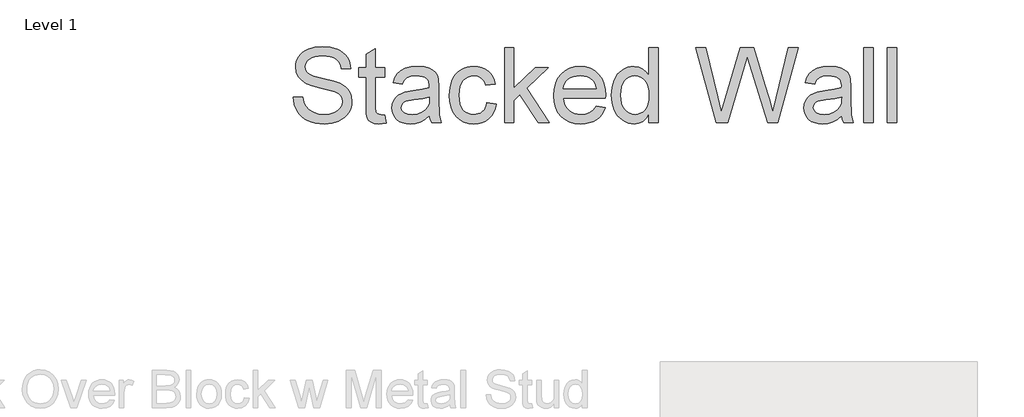
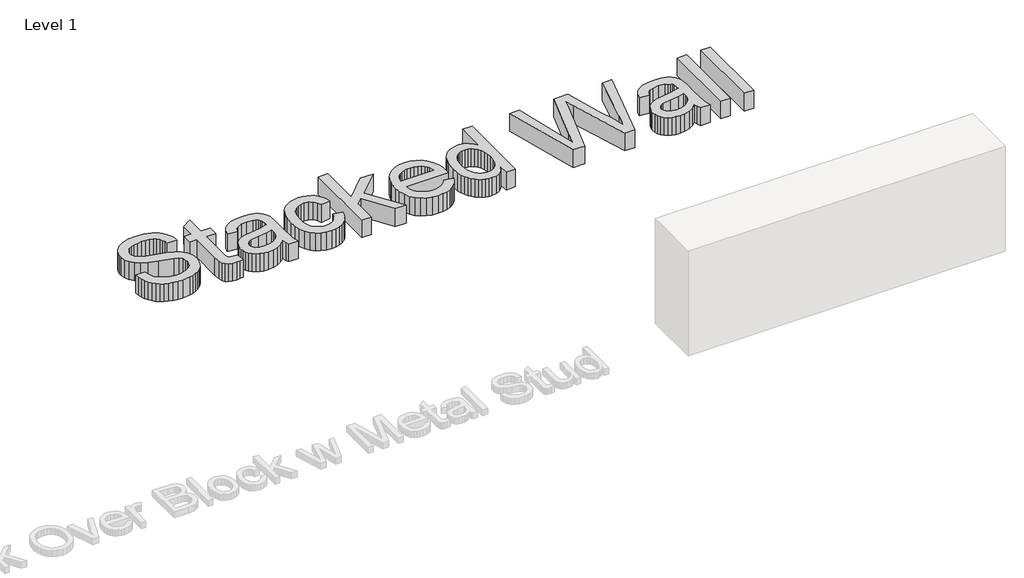
# One storey, part 42 of 42: 1 proxy.
"""IFC4 building model written with IfcOpenShell, lengths in millimetres."""

from ifc_helpers import new_model, si_unit, origin, origin_with_axes, place, context, project, spatial, polyline, outline, extrude, element, save

model = new_model("IFC4")

# Units and contexts
model_context = context("Model", 3, world=origin())
ifc_project = project(units=[si_unit("LENGTHUNIT", "METRE", prefix="MILLI")], contexts=[model_context])

# Site, building, storey
site = spatial("IfcSite", under=ifc_project)
building = spatial("IfcBuilding", under=site)
storey = spatial("IfcBuildingStorey", under=building, Name="Level 1", Elevation=0.0)

# Proxy
placement = place(None, origin())
element("IfcBuildingElementProxy", 1, Name="24\" Arial", ObjectType="24\" Arial", at=placement, inside=storey, context=model_context, shape_type="SweptSolid", body=[
    extrude(outline(polyline([(32520.8544204, 19214.0234856), (32596.9961939, 19214.0234856), (32605.733165, 19171.7700063), (32621.5340701, 19137.8073549), (32646.1834821, 19110.8528696), (32681.4659739, 19089.6238888), (32724.5931503, 19075.8492174), (32772.7766163, 19071.2576603), (32815.1973993, 19074.7338594), (32852.3388211, 19085.1624568), (32882.4348981, 19101.6697554), (32903.7196468, 19123.382058), (32916.3789602, 19148.3103095), (32920.5987313, 19174.4654548), (32917.4385503, 19199.9513854), (32907.9580072, 19221.9797061), (32888.6994922, 19240.7734886), (32856.2053955, 19256.5558044), (32745.3388093, 19285.6294699), (32672.5616991, 19304.8693956), (32625.9955022, 19323.1798562), (32588.0919191, 19348.7959119), (32561.2303803, 19379.8400432), (32545.2249929, 19415.6430353), (32539.8898637, 19455.5356735), (32541.5396641, 19478.2099724), (32546.4890653, 19500.1314046), (32554.7380673, 19521.2999702), (32566.28667, 19541.7156691), (32581.0047484, 19560.5466302), (32598.7621774, 19576.9609822), (32619.558957, 19590.9587253), (32643.3950871, 19602.5398593), (32696.9694502, 19618.0991035), (32756.2693178, 19623.2855183), (32820.5139392, 19617.8574426), (32876.7279829, 19601.5732157), (32901.321627, 19589.4436973), (32922.9038046, 19574.7674448), (32941.4745154, 19557.5444582), (32957.0337597, 19537.7747375), (32969.4607068, 19516.0345509), (32978.6345265, 19492.9001668), (32984.5552186, 19468.3715853), (32987.2227832, 19442.4488062), (32911.0810096, 19442.4488062), (32905.9875414, 19466.7450215), (32897.1018559, 19487.8810558), (32884.4239532, 19505.8569091), (32867.9538332, 19520.6725813), (32847.3847726, 19532.2537153), (32822.4100478, 19540.5259539), (32793.0296589, 19545.489297), (32759.2436058, 19547.1437447), (32724.3793733, 19545.5078863), (32694.5900198, 19540.6003111), (32669.8755452, 19532.421019), (32650.2359496, 19520.9700101), (32635.2715629, 19507.2046333), (32624.5827153, 19492.0822376), (32618.1694068, 19475.602823), (32616.0316373, 19457.7663895), (32617.5466652, 19442.4209222), (32622.0917491, 19428.506831), (32629.6668889, 19416.024116), (32640.2720847, 19404.972777), (32656.9652762, 19394.507001), (32683.2505467, 19383.9296892), (32764.5973243, 19362.4404582), (32848.5466039, 19342.0294066), (32899.3325719, 19324.2208571), (32942.7385878, 19296.597157), (32959.5200786, 19280.3594033), (32973.0205578, 19262.5043805), (32983.3980346, 19243.125035), (32990.8105181, 19222.3143135), (32996.7405048, 19176.3987421), (32995.0349366, 19152.5812012), (32989.9182317, 19129.4607591), (32981.3903902, 19107.0374158), (32969.4514122, 19085.3111712), (32954.3104272, 19065.1231912), (32936.1765649, 19047.3146416), (32915.0498252, 19031.8855225), (32890.9302082, 19018.8358338), (32864.51946, 19008.458357), (32836.5193266, 19001.0458735), (32775.7509044, 18995.1158868), (32736.8016732, 18996.7145666), (32701.1520428, 19001.510606), (32668.8020131, 19009.5040051), (32639.7515843, 19020.6947638), (32613.8241579, 19035.1014714), (32590.8431355, 19052.7427173), (32570.8085173, 19073.6185014), (32553.7203031, 19097.7288237), (32539.9549263, 19124.2929337), (32529.8888202, 19152.5300806), (32523.5219849, 19182.4402646), (32520.8544204, 19214.0234856)])), origin_with_axes(), (0.0, 0.0, 1.0), 152.4),
    extrude(outline(polyline([(33263.2367122, 19068.1346578), (33272.7544338, 19002.4028924), (33242.602589, 18996.9376382), (33215.7968181, 18995.1158868), (33179.250254, 18998.2760678), (33151.9983399, 19007.7566109), (33132.7398249, 19022.3678008), (33120.173458, 19040.9199224), (33113.2582383, 19072.7819829), (33110.9531651, 19127.3229896), (33110.9531651, 19375.8247543), (33053.846835, 19375.8247543), (33053.846835, 19451.9665279), (33110.9531651, 19451.9665279), (33110.9531651, 19560.6767553), (33187.0949386, 19605.4397901), (33187.0949386, 19451.9665279), (33263.2367122, 19451.9665279), (33263.2367122, 19375.8247543), (33187.0949386, 19375.8247543), (33187.0949386, 19129.5537056), (33191.1102275, 19090.2931036), (33204.1227376, 19076.3883071), (33215.109014, 19072.540322), (33230.0734006, 19071.2576603), (33263.2367122, 19068.1346578)])), origin_with_axes(), (0.0, 0.0, 1.0), 152.4),
    extrude(outline(polyline([(33624.9101364, 19061.7399386), (33588.5308759, 19030.5470929), (33551.0734361, 19010.1360413), (33511.682709, 18998.8709254), (33469.5035869, 18995.1158868), (33435.6013507, 18997.3744867), (33405.8724124, 19004.1502866), (33380.316772, 19015.4432865), (33358.9344295, 19031.2534863), (33342.0506976, 19050.5770638), (33329.9908891, 19072.4101969), (33322.755004, 19096.7528855), (33320.3430423, 19123.6051296), (33323.9865451, 19155.1697613), (33334.9170536, 19183.8344621), (33351.7775489, 19208.3723384), (33373.211012, 19227.5564961), (33398.3995137, 19242.0561503), (33426.5251249, 19252.5405156), (33492.4056047, 19263.9915245), (33570.2575938, 19276.037391), (33624.4639932, 19290.1652591), (33624.9101364, 19307.1187009), (33619.6679537, 19341.0999416), (33613.1152254, 19353.6848978), (33603.9414058, 19363.3327446), (33588.0847327, 19372.9620021), (33568.7704498, 19379.8400432), (33519.7690546, 19385.342476), (33474.4111621, 19381.6803839), (33442.7349946, 19370.6941075), (33421.1342278, 19350.3760024), (33406.0025375, 19318.7184242), (33329.860764, 19328.2361459), (33343.0777564, 19369.8761783), (33362.8010039, 19402.5933466), (33390.8708472, 19427.6145446), (33429.1276269, 19446.1666662), (33475.9168955, 19457.6548537), (33529.5842051, 19461.4842495), (33581.0579772, 19458.1009969), (33621.8614911, 19447.951239), (33652.6267829, 19432.6894236), (33673.9858888, 19413.9699983), (33688.1509356, 19390.8263196), (33697.3340498, 19362.2917438), (33701.0519099, 19295.667692), (33701.0519099, 19200.9366183), (33704.9184843, 19068.6551582), (33710.6439888, 19035.9565792), (33720.0873533, 19004.6336084), (33643.9455797, 19004.6336084), (33631.7509988, 19031.1047719), (33624.9101364, 19061.7399386)]), holes=[polyline([(33624.9101364, 19214.0234856), (33573.7523823, 19201.3455829), (33502.0720408, 19190.6753246), (33436.563347, 19178.3320293), (33419.5169587, 19169.892487), (33406.8948239, 19158.2555851), (33399.0873178, 19144.31361), (33396.4848158, 19128.958848), (33402.1545524, 19106.3170804), (33419.163762, 19087.7649588), (33447.1406588, 19075.3844849), (33485.7134567, 19071.2576603), (33526.609917, 19075.8120388), (33562.7475166, 19089.4751744), (33592.0442537, 19109.6073865), (33612.4181266, 19133.5689945), (33621.4525265, 19158.2555851), (33624.4639932, 19192.4598974), (33624.9101364, 19214.0234856)])]), origin_with_axes(), (0.0, 0.0, 1.0), 152.4),
    extrude(outline(polyline([(34091.2784992, 19166.4348772), (34167.4202727, 19156.9171555), (34159.1387394, 19120.9886856), (34146.1912919, 19089.1963349), (34128.57793, 19061.5401036), (34106.2986537, 19038.0199916), (34080.2922228, 19019.2494457), (34051.4973968, 19005.841913), (34019.9141758, 18997.7973933), (33985.5425598, 18995.1158868), (33942.8382899, 18998.8569834), (33904.5489789, 19010.0802734), (33870.6746267, 19028.7857567), (33841.2152332, 19054.9734333), (33817.3698084, 19088.1506868), (33800.3373621, 19127.8249007), (33790.1178943, 19173.996075), (33786.7114051, 19226.6642097), (33792.529856, 19294.4222089), (33799.8029197, 19324.9133085), (33809.9852089, 19353.1458081), (33823.1464334, 19378.5527341), (33839.3563032, 19400.5671129), (33858.6148182, 19419.1889443), (33880.9219784, 19434.4182285), (33905.2693143, 19446.2596127), (33930.6483563, 19454.7177443), (33957.0591046, 19459.7926232), (33984.5015589, 19461.4842495), (34018.2829647, 19459.160587), (34048.8391269, 19452.1895995), (34076.1700454, 19440.5712868), (34100.2757204, 19424.3056492), (34120.7471873, 19403.7644725), (34137.1754813, 19379.3195428), (34149.5606025, 19350.97086), (34157.902551, 19318.7184242), (34081.7607775, 19309.2007025), (34067.9489274, 19342.4197819), (34046.4411071, 19366.2326754), (34018.4270318, 19380.5650259), (33985.0964166, 19385.342476), (33959.224758, 19382.9909296), (33935.890539, 19375.9362901), (33915.0937594, 19364.1785578), (33896.8344193, 19347.7177325), (33881.9676265, 19326.1727336), (33871.3484888, 19299.1624804), (33864.9770061, 19266.686973), (33862.8531786, 19228.7462114), (33864.9305329, 19190.2338287), (33871.1625958, 19157.381888), (33881.5493673, 19130.1903891), (33896.0908473, 19108.6593322), (33913.9876961, 19092.2961007), (33934.4405736, 19080.6080783), (33957.4494799, 19073.5952648), (33983.0144149, 19071.2576603), (34022.4423206, 19077.0947005), (34039.4933562, 19084.3910008), (34054.7691136, 19094.6058213), (34067.842039, 19107.8506977), (34078.2845783, 19124.2371658), (34086.0967317, 19143.7652256), (34091.2784992, 19166.4348772)])), origin_with_axes(), (0.0, 0.0, 1.0), 152.4),
    extrude(outline(polyline([(34234.0443245, 19004.6336084), (34234.0443245, 19613.7677966), (34310.186098, 19613.7677966), (34310.186098, 19286.4473991), (34480.9102308, 19451.9665279), (34586.200027, 19451.9665279), (34413.3938926, 19284.3653975), (34595.7177487, 19004.6336084), (34506.7865367, 19004.6336084), (34358.8157073, 19231.4230706), (34310.186098, 19184.2806053), (34310.186098, 19004.6336084), (34234.0443245, 19004.6336084)])), origin_with_axes(), (0.0, 0.0, 1.0), 152.4),
    extrude(outline(polyline([(34975.5343299, 19137.8817121), (35050.1889594, 19128.3639904), (35038.7425978, 19098.4631011), (35023.290242, 19072.1127681), (35003.8318921, 19049.3129914), (34980.3675479, 19030.0637711), (34953.1388705, 19014.7740717), (34922.3875207, 19003.8528578), (34888.1134985, 18997.3001295), (34850.3168039, 18995.1158868), (34803.0720975, 18998.8848674), (34760.9766273, 19010.1918092), (34724.0303932, 19029.0367122), (34692.2333952, 19055.4195765), (34666.6638128, 19088.6061247), (34648.3998254, 19127.8620793), (34637.4414329, 19173.1874405), (34633.7886355, 19224.5822081), (34637.4786115, 19277.7197227), (34648.5485398, 19324.5554645), (34666.9984202, 19365.0894335), (34692.8282528, 19399.3216298), (34724.5415989, 19426.5177759), (34760.6420199, 19445.9435946), (34801.1295156, 19457.5990858), (34846.0040863, 19461.4842495), (34889.4333388, 19457.6083805), (34928.7078827, 19445.9807732), (34963.8277181, 19426.6014278), (34994.7928449, 19399.4703442), (35020.0696458, 19365.3125051), (35038.1245036, 19324.8528933), (35048.9574182, 19278.0915087), (35052.5683898, 19225.0283513), (35052.1222466, 19204.5057639), (34709.930409, 19204.5057639), (34714.3407204, 19174.1215528), (34723.1102228, 19147.5109696), (34736.2389161, 19124.6740143), (34753.7268002, 19105.610687), (34774.6072316, 19090.5812378), (34797.9135667, 19079.8459169), (34823.6458055, 19073.4047244), (34851.8039479, 19071.2576603), (34892.3286223, 19075.2357705), (34926.4585774, 19087.1701012), (34954.1938133, 19107.8042244), (34975.5343299, 19137.8817121)]), holes=[polyline([(34709.930409, 19280.6475374), (34976.4266163, 19280.6475374), (34966.128144, 19320.874783), (34957.2703425, 19336.6942775), (34945.940164, 19349.6510197), (34925.1759157, 19365.2660318), (34901.5489152, 19376.4196119), (34875.0591624, 19383.11176), (34845.7066575, 19385.342476), (34818.9334179, 19383.5625505), (34794.3815997, 19378.2227741), (34772.0512028, 19369.3231466), (34751.9422274, 19356.8636682), (34735.0677901, 19341.420607), (34722.441008, 19323.5702315), (34714.0618809, 19303.3125417), (34709.930409, 19280.6475374)])]), origin_with_axes(), (0.0, 0.0, 1.0), 152.4),
    extrude(outline(polyline([(35404.7240923, 19004.6336084), (35404.7240923, 19076.4626643), (35381.942905, 19040.8734491), (35354.3470888, 19015.4525811), (35321.936644, 19000.2000603), (35284.7115704, 18995.1158868), (35259.5788366, 18996.9562275), (35235.4871035, 19002.4772496), (35212.4363713, 19011.6789532), (35190.4266399, 19024.5613382), (35170.1457134, 19040.7386767), (35152.2813959, 19059.8252407), (35136.8336875, 19081.8210301), (35123.8025881, 19106.726045), (35113.4576425, 19134.0662582), (35106.0683957, 19163.3676426), (35100.1569983, 19227.8539249), (35105.6036632, 19291.5408673), (35121.9436581, 19349.0561621), (35134.1940069, 19374.6815124), (35149.1583935, 19397.1280923), (35166.836818, 19416.395902), (35187.2292803, 19432.4849413), (35209.615445, 19445.1721386), (35233.2749768, 19454.2344225), (35258.2078757, 19459.6717928), (35284.4141416, 19461.4842495), (35321.6670991, 19456.2978348), (35354.6073391, 19440.7385905), (35382.5284679, 19416.8885184), (35404.7240923, 19386.82962), (35404.7240923, 19613.7677966), (35480.8658658, 19613.7677966), (35480.8658658, 19004.6336084), (35404.7240923, 19004.6336084)]), holes=[polyline([(35176.2987718, 19228.1513537), (35178.4458359, 19191.2283563), (35184.8870285, 19159.2779966), (35195.6223493, 19132.3002747), (35210.6517985, 19110.2951906), (35228.5997678, 19093.2162711), (35248.090649, 19081.0170429), (35269.1244422, 19073.6975059), (35291.7011473, 19071.2576603), (35314.3847408, 19073.5859701), (35335.2930562, 19080.5708997), (35354.4260934, 19092.2124489), (35371.7838524, 19108.5106178), (35386.1952074, 19129.5955315), (35396.4890323, 19155.5973152), (35402.6653273, 19186.5159687), (35404.7240923, 19222.3514921), (35402.6281487, 19261.639978), (35396.3403179, 19295.3330846), (35385.8606, 19323.4308118), (35371.1889948, 19345.9331597), (35353.4501551, 19363.1747356), (35333.7687336, 19375.4901469), (35312.1447301, 19382.8793938), (35288.5781448, 19385.342476), (35265.5552966, 19382.9769876), (35244.5215034, 19375.8805222), (35225.4767654, 19364.05308), (35208.4210825, 19347.4946609), (35194.3675715, 19325.8427735), (35184.3293494, 19298.7349265), (35178.3064162, 19266.1711199), (35176.2987718, 19228.1513537)])]), origin_with_axes(), (0.0, 0.0, 1.0), 152.4),
    extrude(outline(polyline([(35951.5469463, 19004.6336084), (35785.4329599, 19613.7677966), (35863.9541638, 19613.7677966), (35960.321096, 19213.428628), (35990.0639762, 19089.8469604), (36021.8888581, 19199.1520455), (36142.6449521, 19613.7677966), (36255.8166115, 19613.7677966), (36343.5581084, 19313.2159913), (36381.1456733, 19201.6801903), (36408.8437306, 19089.8469604), (36437.6943245, 19209.8594824), (36534.953543, 19613.7677966), (36613.4747469, 19613.7677966), (36447.2120461, 19004.6336084), (36365.8652686, 19004.6336084), (36219.8277264, 19474.5711169), (36199.4538534, 19540.1541679), (36176.5518356, 19461.1868207), (36043.4524463, 19004.6336084), (35951.5469463, 19004.6336084)])), origin_with_axes(), (0.0, 0.0, 1.0), 152.4),
    extrude(outline(polyline([(36965.6304494, 19061.7399386), (36929.251189, 19030.5470929), (36891.7937491, 19010.1360413), (36852.4030221, 18998.8709254), (36810.2239, 18995.1158868), (36776.3216638, 18997.3744867), (36746.5927255, 19004.1502866), (36721.037085, 19015.4432865), (36699.6547425, 19031.2534863), (36682.7710106, 19050.5770638), (36670.7112021, 19072.4101969), (36663.4753171, 19096.7528855), (36661.0633554, 19123.6051296), (36664.7068582, 19155.1697613), (36675.6373667, 19183.8344621), (36692.497862, 19208.3723384), (36713.9313251, 19227.5564961), (36739.1198268, 19242.0561503), (36767.245438, 19252.5405156), (36833.1259178, 19263.9915245), (36910.9779069, 19276.037391), (36965.1843062, 19290.1652591), (36965.6304494, 19307.1187009), (36960.3882668, 19341.0999416), (36953.8355385, 19353.6848978), (36944.6617188, 19363.3327446), (36928.8050458, 19372.9620021), (36909.4907629, 19379.8400432), (36860.4893676, 19385.342476), (36815.1314752, 19381.6803839), (36783.4553077, 19370.6941075), (36761.8545409, 19350.3760024), (36746.7228506, 19318.7184242), (36670.581077, 19328.2361459), (36683.7980695, 19369.8761783), (36703.521317, 19402.5933466), (36731.5911602, 19427.6145446), (36769.84794, 19446.1666662), (36816.6372085, 19457.6548537), (36870.3045181, 19461.4842495), (36921.7782903, 19458.1009969), (36962.5818042, 19447.951239), (36993.347096, 19432.6894236), (37014.7062019, 19413.9699983), (37028.8712486, 19390.8263196), (37038.0543629, 19362.2917438), (37041.7722229, 19295.667692), (37041.7722229, 19200.9366183), (37045.6387974, 19068.6551582), (37051.3643018, 19035.9565792), (37060.8076663, 19004.6336084), (36984.6658928, 19004.6336084), (36972.4713119, 19031.1047719), (36965.6304494, 19061.7399386)]), holes=[polyline([(36965.6304494, 19214.0234856), (36914.4726953, 19201.3455829), (36842.7923539, 19190.6753246), (36777.28366, 19178.3320293), (36760.2372718, 19169.892487), (36747.615137, 19158.2555851), (36739.8076309, 19144.31361), (36737.2051289, 19128.958848), (36742.8748654, 19106.3170804), (36759.8840751, 19087.7649588), (36787.8609718, 19075.3844849), (36826.4337697, 19071.2576603), (36867.3302301, 19075.8120388), (36903.4678296, 19089.4751744), (36932.7645667, 19109.6073865), (36953.1384397, 19133.5689945), (36962.1728396, 19158.2555851), (36965.1843062, 19192.4598974), (36965.6304494, 19214.0234856)])]), origin_with_axes(), (0.0, 0.0, 1.0), 152.4),
    extrude(outline(polyline([(37146.4671615, 19004.6336084), (37146.4671615, 19613.7677966), (37222.608935, 19613.7677966), (37222.608935, 19004.6336084), (37146.4671615, 19004.6336084)])), origin_with_axes(), (0.0, 0.0, 1.0), 152.4),
    extrude(outline(polyline([(37336.8215953, 19004.6336084), (37336.8215953, 19613.7677966), (37412.9633688, 19613.7677966), (37412.9633688, 19004.6336084), (37336.8215953, 19004.6336084)])), origin_with_axes(), (0.0, 0.0, 1.0), 152.4),
])

save(model, "model.ifc")

# Revit data of these elements
# Element 1 (IfcBuildingElementProxy, "24\" Arial")
#   Phase Created = New Construction
